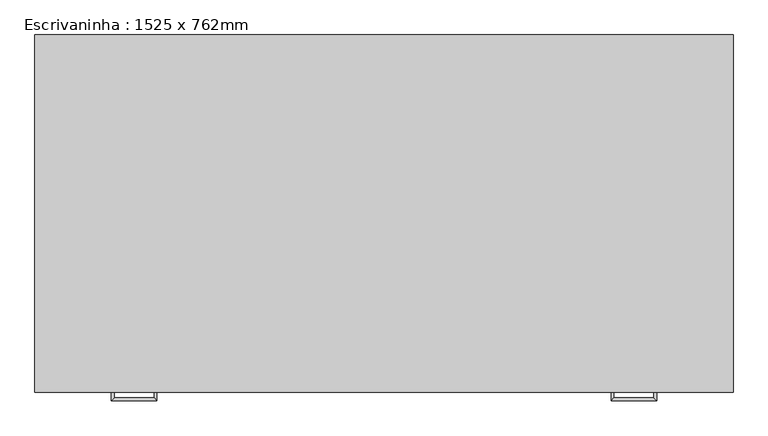
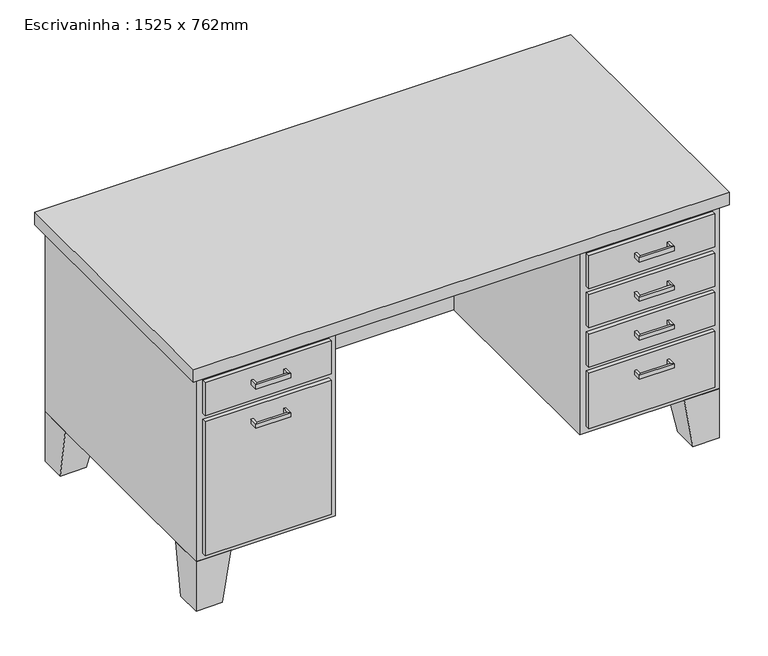
"""IFC4 building model written with IfcOpenShell, lengths in millimetres: furniture geometry, Escrivaninha : 1525 x 762mm."""

from ifc_helpers import new_model, si_unit, frame, origin, place, context, project, spatial, polyline, outline, extrude, faceted_brep, source, transform, mapped, element, save


def escrivaninha_1525_x_762mm_8f660baf(model_context):
    return source(origin(), model_context, "Body", "SolidModel", [
        extrude(outline(polyline([(18.55, 0.0), (386.85, 0.0), (386.85, -12.7), (18.55, -12.7), (18.55, 0.0)])), frame((0.0, 0.0, 603.25), z_axis=(0.0, 0.0, 1.0), x_axis=(1.0, 0.0, 0.0)), (0.0, 0.0, 1.0), 101.6),
        extrude(outline(polyline([(18.55, 0.0), (386.85, 0.0), (386.85, -12.7), (18.55, -12.7), (18.55, 0.0)])), frame((0.0, 0.0, 171.05), z_axis=(0.0, 0.0, 1.0), x_axis=(1.0, 0.0, 0.0)), (0.0, 0.0, 1.0), 413.15),
        extrude(outline(polyline([(1137.15, 0.0), (1505.45, 0.0), (1505.45, -12.7), (1137.15, -12.7), (1137.15, 0.0)])), frame((0.0, 0.0, 602.85), z_axis=(0.0, 0.0, 1.0), x_axis=(1.0, 0.0, 0.0)), (0.0, 0.0, 1.0), 102.0),
        extrude(outline(polyline([(1137.15, 0.0), (1505.45, 0.0), (1505.45, -12.7), (1137.15, -12.7), (1137.15, 0.0)])), frame((0.0, 0.0, 171.05), z_axis=(0.0, 0.0, 1.0), x_axis=(1.0, 0.0, 0.0)), (0.0, 0.0, 1.0), 171.45),
        extrude(outline(polyline([(1137.15, 0.0), (1505.45, 0.0), (1505.45, -12.7), (1137.15, -12.7), (1137.15, 0.0)])), frame((0.0, 0.0, 482.2), z_axis=(0.0, 0.0, 1.0), x_axis=(1.0, 0.0, 0.0)), (0.0, 0.0, 1.0), 101.6),
        extrude(outline(polyline([(1137.15, 0.0), (1505.45, 0.0), (1505.45, -12.7), (1137.15, -12.7), (1137.15, 0.0)])), frame((0.0, 0.0, 361.55), z_axis=(0.0, 0.0, 1.0), x_axis=(1.0, 0.0, 0.0)), (0.0, 0.0, 1.0), 101.6),
        faceted_brep([(101.1, 0.0, 152.0), (101.1, 101.6, 152.0), (-0.5, 101.6, 152.0), (-0.5, 0.0, 152.0), (75.7, 0.0, 0.0), (-0.5, 0.0, 0.0), (-0.5, 76.2, 0.0), (75.7, 76.2, 0.0)], [[[0, 1, 2, 3]], [[4, 5, 6, 7]], [[4, 7, 1, 0]], [[7, 6, 2, 1]], [[6, 5, 3, 2]], [[5, 4, 0, 3]]]),
        faceted_brep([(101.1, 762.0, 152.0), (-0.5, 762.0, 152.0), (-0.5, 660.4, 152.0), (101.1, 660.4, 152.0), (75.7, 762.0, 0.0), (75.7, 685.8, 0.0), (-0.5, 685.8, 0.0), (-0.5, 762.0, 0.0)], [[[0, 1, 2, 3]], [[4, 5, 6, 7]], [[4, 7, 1, 0]], [[7, 6, 2, 1]], [[6, 5, 3, 2]], [[5, 4, 0, 3]]]),
        faceted_brep([(1422.9, 762.0, 152.0), (1422.9, 660.4, 152.0), (1524.5, 660.4, 152.0), (1524.5, 762.0, 152.0), (1448.3, 762.0, 0.0), (1524.5, 762.0, 0.0), (1524.5, 685.8, 0.0), (1448.3, 685.8, 0.0)], [[[0, 1, 2, 3]], [[4, 5, 6, 7]], [[4, 7, 1, 0]], [[7, 6, 2, 1]], [[6, 5, 3, 2]], [[5, 4, 0, 3]]]),
        faceted_brep([(1422.9, 0.0, 152.0), (1524.5, 0.0, 152.0), (1524.5, 101.6, 152.0), (1422.9, 101.6, 152.0), (1448.3, 0.0, 0.0), (1448.3, 76.2, 0.0), (1524.5, 76.2, 0.0), (1524.5, 0.0, 0.0)], [[[0, 1, 2, 3]], [[4, 5, 6, 7]], [[4, 7, 1, 0]], [[7, 6, 2, 1]], [[6, 5, 3, 2]], [[5, 4, 0, 3]]]),
        extrude(outline(polyline([(-19.55, -19.05), (-19.55, 781.05), (1543.55, 781.05), (1543.55, -19.05), (-19.55, -19.05)])), frame((0.0, 0.0, 723.9), z_axis=(0.0, 0.0, 1.0), x_axis=(1.0, 0.0, 0.0)), (0.0, 0.0, 1.0), 38.1),
        extrude(outline(polyline([(1118.1, 0.0), (1118.1, 635.0), (405.9, 635.0), (405.9, 0.0), (-0.5, 0.0), (-0.5, 762.0), (1524.5, 762.0), (1524.5, 0.0), (1118.1, 0.0)])), frame((0.0, 0.0, 152.0), z_axis=(0.0, 0.0, 1.0), x_axis=(1.0, 0.0, 0.0)), (0.0, 0.0, 1.0), 571.9),
        faceted_brep([(158.25, -12.7, 546.1), (158.25, -12.7, 533.4), (151.9, -12.7, 533.4), (151.9, -12.7, 546.1), (158.25, -31.75, 546.1), (158.25, -31.75, 533.4), (151.9, -38.1, 533.4), (151.9, -38.1, 546.1), (247.15, -31.75, 546.1), (247.15, -31.75, 533.4), (253.5, -38.1, 533.4), (253.5, -38.1, 546.1), (247.15, -12.7, 546.1), (253.5, -12.7, 546.1), (253.5, -12.7, 533.4), (247.15, -12.7, 533.4)], [[[0, 1, 2, 3]], [[1, 0, 4, 5]], [[2, 1, 5, 6]], [[3, 2, 6, 7]], [[0, 3, 7, 4]], [[5, 4, 8, 9]], [[6, 5, 9, 10]], [[7, 6, 10, 11]], [[4, 7, 11, 8]], [[12, 13, 14, 15]], [[9, 8, 12, 15]], [[10, 9, 15, 14]], [[11, 10, 14, 13]], [[8, 11, 13, 12]]]),
        faceted_brep([(158.25, -12.7, 666.75), (158.25, -12.7, 654.05), (151.9, -12.7, 654.05), (151.9, -12.7, 666.75), (158.25, -31.75, 666.75), (158.25, -31.75, 654.05), (151.9, -38.1, 654.05), (151.9, -38.1, 666.75), (247.15, -31.75, 666.75), (247.15, -31.75, 654.05), (253.5, -38.1, 654.05), (253.5, -38.1, 666.75), (247.15, -12.7, 666.75), (253.5, -12.7, 666.75), (253.5, -12.7, 654.05), (247.15, -12.7, 654.05)], [[[0, 1, 2, 3]], [[1, 0, 4, 5]], [[2, 1, 5, 6]], [[3, 2, 6, 7]], [[0, 3, 7, 4]], [[5, 4, 8, 9]], [[6, 5, 9, 10]], [[7, 6, 10, 11]], [[4, 7, 11, 8]], [[12, 13, 14, 15]], [[9, 8, 12, 15]], [[10, 9, 15, 14]], [[11, 10, 14, 13]], [[8, 11, 13, 12]]]),
        faceted_brep([(1365.75, -12.7, 304.8), (1372.1, -12.7, 304.8), (1372.1, -12.7, 292.1), (1365.75, -12.7, 292.1), (1365.75, -31.75, 304.8), (1372.1, -38.1, 304.8), (1372.1, -38.1, 292.1), (1365.75, -31.75, 292.1), (1276.85, -31.75, 304.8), (1270.5, -38.1, 304.8), (1270.5, -38.1, 292.1), (1276.85, -31.75, 292.1), (1276.85, -12.7, 304.8), (1276.85, -12.7, 292.1), (1270.5, -12.7, 292.1), (1270.5, -12.7, 304.8)], [[[0, 1, 2, 3]], [[1, 0, 4, 5]], [[2, 1, 5, 6]], [[3, 2, 6, 7]], [[0, 3, 7, 4]], [[5, 4, 8, 9]], [[6, 5, 9, 10]], [[7, 6, 10, 11]], [[4, 7, 11, 8]], [[12, 13, 14, 15]], [[9, 8, 12, 15]], [[10, 9, 15, 14]], [[11, 10, 14, 13]], [[8, 11, 13, 12]]]),
        faceted_brep([(1365.75, -12.7, 425.45), (1372.1, -12.7, 425.45), (1372.1, -12.7, 412.75), (1365.75, -12.7, 412.75), (1365.75, -31.75, 425.45), (1372.1, -38.1, 425.45), (1372.1, -38.1, 412.75), (1365.75, -31.75, 412.75), (1276.85, -31.75, 425.45), (1270.5, -38.1, 425.45), (1270.5, -38.1, 412.75), (1276.85, -31.75, 412.75), (1276.85, -12.7, 425.45), (1276.85, -12.7, 412.75), (1270.5, -12.7, 412.75), (1270.5, -12.7, 425.45)], [[[0, 1, 2, 3]], [[1, 0, 4, 5]], [[2, 1, 5, 6]], [[3, 2, 6, 7]], [[0, 3, 7, 4]], [[5, 4, 8, 9]], [[6, 5, 9, 10]], [[7, 6, 10, 11]], [[4, 7, 11, 8]], [[12, 13, 14, 15]], [[9, 8, 12, 15]], [[10, 9, 15, 14]], [[11, 10, 14, 13]], [[8, 11, 13, 12]]]),
        faceted_brep([(1365.75, -12.7, 546.1), (1372.1, -12.7, 546.1), (1372.1, -12.7, 533.4), (1365.75, -12.7, 533.4), (1365.75, -31.75, 546.1), (1372.1, -38.1, 546.1), (1372.1, -38.1, 533.4), (1365.75, -31.75, 533.4), (1276.85, -31.75, 546.1), (1270.5, -38.1, 546.1), (1270.5, -38.1, 533.4), (1276.85, -31.75, 533.4), (1276.85, -12.7, 546.1), (1276.85, -12.7, 533.4), (1270.5, -12.7, 533.4), (1270.5, -12.7, 546.1)], [[[0, 1, 2, 3]], [[1, 0, 4, 5]], [[2, 1, 5, 6]], [[3, 2, 6, 7]], [[0, 3, 7, 4]], [[5, 4, 8, 9]], [[6, 5, 9, 10]], [[7, 6, 10, 11]], [[4, 7, 11, 8]], [[12, 13, 14, 15]], [[9, 8, 12, 15]], [[10, 9, 15, 14]], [[11, 10, 14, 13]], [[8, 11, 13, 12]]]),
        faceted_brep([(1365.75, -12.7, 666.75), (1372.1, -12.7, 666.75), (1372.1, -12.7, 654.05), (1365.75, -12.7, 654.05), (1365.75, -31.75, 666.75), (1372.1, -38.1, 666.75), (1372.1, -38.1, 654.05), (1365.75, -31.75, 654.05), (1276.85, -31.75, 666.75), (1270.5, -38.1, 666.75), (1270.5, -38.1, 654.05), (1276.85, -31.75, 654.05), (1276.85, -12.7, 666.75), (1276.85, -12.7, 654.05), (1270.5, -12.7, 654.05), (1270.5, -12.7, 666.75)], [[[0, 1, 2, 3]], [[1, 0, 4, 5]], [[2, 1, 5, 6]], [[3, 2, 6, 7]], [[0, 3, 7, 4]], [[5, 4, 8, 9]], [[6, 5, 9, 10]], [[7, 6, 10, 11]], [[4, 7, 11, 8]], [[12, 13, 14, 15]], [[9, 8, 12, 15]], [[10, 9, 15, 14]], [[11, 10, 14, 13]], [[8, 11, 13, 12]]]),
    ])


if __name__ == "__main__":
    model = new_model("IFC4")
    model_context = context("Model", 3, world=origin())
    ifc_project = project(units=[si_unit("LENGTHUNIT", "METRE", prefix="MILLI")], contexts=[model_context])
    site = spatial("IfcSite", under=ifc_project)
    building = spatial("IfcBuilding", under=site)
    placement = place(None, origin())
    escrivaninha_1525_x_762mm_shape = escrivaninha_1525_x_762mm_8f660baf(model_context)
    element("IfcFurniture", 1, ObjectType="Escrivaninha : 1525 x 762mm", at=placement, inside=building, context=model_context, shape_type="MappedRepresentation", body=[
        mapped(escrivaninha_1525_x_762mm_shape, transform((0.0, 0.0, 0.0), x_axis=(1.0, 0.0, 0.0), y_axis=(0.0, 1.0, 0.0), z_axis=(0.0, 0.0, 1.0))),
    ])
    save(model, "model.ifc")

# Revit data of these elements
# Type "Escrivaninha : 1525 x 762mm"
#   Linear = 762 mm
#   Altura = 762 mm
#   Altura da perna = 152 mm
#   Largura = 1525 mm
#   Material do corpo = Laminado - Marfim, Fosco
#   Material Puxador/Perna = Aço, Cromo polido
#   Material superior = Cerejeira
#   Assembly Code = ""
# Element 1 (IfcFurniture, "Escrivaninha : 1525 x 762mm")
#   Materials on its faces: "Aço, Cromo polido", "Laminado - Marfim, Fosco", "Cerejeira"
# Materials
#   "Laminado - Marfim, Fosco": class "Plástico", colour RGB 247 247 239, transparency 0, Description = "Laminado plástico - Marfim, Fosco", Cost = 0
#   "Aço, Cromo polido": class "Metal", colour RGB 17 17 17, transparency 0, Description = "Aço revestido de cromo", Cost = 0
#   "Cerejeira": class "Madeira", colour RGB 226 177 128, transparency 0, Description = "Prunus Serotina", Cost = 0
